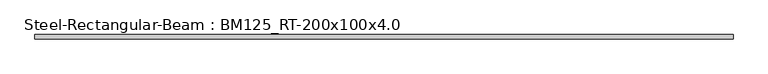
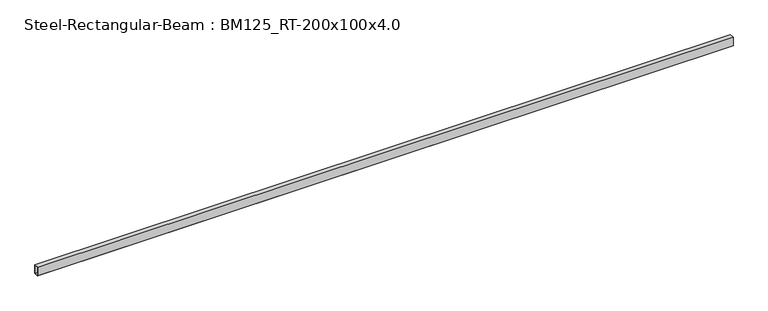
"""IFC4 building model written with IfcOpenShell, lengths in millimetres: beam geometry, Steel-Rectangular-Beam : BM125_RT-200x100x4.0."""

import ifcopenshell
import ifcopenshell.guid

model = None  # the IFC model being written
_history = None  # IfcOwnerHistory: only IFC2X3 demands one
_inside = {}  # id of a spatial element -> (the spatial element, [elements in it])
_under = {}  # id of a project, library or spatial element -> (it, [spatial elements below it])
_declared = {}  # id of a project -> (the project, [libraries it declares])
_typed = {}  # id of a type object -> (the type object, [elements of that type])
_made_of = {}  # id of a material, layer set ... -> (it, [elements and type objects made of it])


def new_model(schema):
    """Start an empty IFC model of exactly this schema.

    Asked for "IFC4X3", IfcOpenShell would pick the latest addendum, in which some entities
    have other attributes; the version numbers below select the first issue.
    IFC2X3 requires an IfcOwnerHistory on every rooted entity: one is made here for all.
    """
    global model, _history
    if schema == "IFC4X3":
        model = ifcopenshell.file(schema_version=(4, 3, 0, 0))
    else:
        model = ifcopenshell.file(schema=schema)
    _inside.clear()
    _under.clear()
    _declared.clear()
    _typed.clear()
    _made_of.clear()
    _history = None
    if model.schema == "IFC2X3":
        org = make("IfcOrganization", Name="unknown")
        user = make(
            "IfcPersonAndOrganization",
            ThePerson=make("IfcPerson", FamilyName="unknown"),
            TheOrganization=org,
        )
        app = make(
            "IfcApplication",
            ApplicationDeveloper=org,
            Version="unknown",
            ApplicationFullName="unknown",
            ApplicationIdentifier="unknown",
        )
        _history = make(
            "IfcOwnerHistory",
            OwningUser=user,
            OwningApplication=app,
            ChangeAction="ADDED",
            CreationDate=0,
        )
    return model


def make(cls, **values):
    """One entity of the class cls with the attributes given. An attribute that is None is left unset."""
    return model.create_entity(
        cls, **{name: value for name, value in values.items() if value is not None}
    )


def rooted(cls, **values):
    """An entity with a GlobalId (a new one), such as an element, a storey or a relation."""
    return make(cls, GlobalId=ifcopenshell.guid.new(), OwnerHistory=_history, **values)


def si_unit(unit_type, name, prefix=None):
    """IfcSIUnit, for example si_unit("LENGTHUNIT", "METRE", prefix="MILLI")."""
    return make("IfcSIUnit", UnitType=unit_type, Prefix=prefix, Name=name)


def assignment(units):
    """IfcUnitAssignment: the units of a project."""
    return None if units is None else make("IfcUnitAssignment", Units=units)


def point(xyz):
    """IfcCartesianPoint."""
    return None if xyz is None else make("IfcCartesianPoint", Coordinates=xyz)


def direction(xyz):
    """IfcDirection."""
    return None if xyz is None else make("IfcDirection", DirectionRatios=xyz)


def frame(location, z_axis=None, x_axis=None):
    """IfcAxis2Placement3D, a coordinate frame: its origin and axes. An axis left out is left unset."""
    return make(
        "IfcAxis2Placement3D",
        Location=point(location),
        Axis=direction(z_axis),
        RefDirection=direction(x_axis),
    )


def origin():
    """The frame at (0, 0, 0) with its axes left unset."""
    return frame((0.0, 0.0, 0.0))


def place(relative_to, where):
    """IfcLocalPlacement: puts the frame where relative to a parent placement (None: the world)."""
    return make(
        "IfcLocalPlacement", PlacementRelTo=relative_to, RelativePlacement=where
    )


def context(
    kind, dimensions, precision=None, world=None, true_north=None, identifier=None
):
    """IfcGeometricRepresentationContext, for example the 3D "Model" context."""
    return make(
        "IfcGeometricRepresentationContext",
        ContextIdentifier=identifier,
        ContextType=kind,
        CoordinateSpaceDimension=dimensions,
        Precision=precision,
        WorldCoordinateSystem=world,
        TrueNorth=true_north,
    )


def project(units=None, contexts=None):
    """IfcProject with its units and contexts."""
    return rooted(
        "IfcProject",
        Name="project",
        RepresentationContexts=contexts,
        UnitsInContext=assignment(units),
    )


def spatial(cls, under=None, at=None, **own):
    """A site, building, storey or space (cls), placed at a placement, below another one or the project."""
    s = rooted(cls, ObjectPlacement=at, **own)
    if under is not None:
        _under.setdefault(under.id(), (under, []))[1].append(s)
    return s


def polyline(points):
    """IfcPolyline through the points."""
    return make("IfcPolyline", Points=[point(p) for p in points])


def outline(outer, holes=None, kind="AREA"):
    """IfcArbitraryClosedProfileDef: a profile drawn as a closed curve; with holes, ...WithVoids."""
    if holes is None:
        return make("IfcArbitraryClosedProfileDef", ProfileType=kind, OuterCurve=outer)
    return make(
        "IfcArbitraryProfileDefWithVoids",
        ProfileType=kind,
        OuterCurve=outer,
        InnerCurves=holes,
    )


def extrude(swept, where, along, depth):
    """IfcExtrudedAreaSolid: the profile swept, set in the frame where, extruded along a direction by depth."""
    return make(
        "IfcExtrudedAreaSolid",
        SweptArea=swept,
        Position=where,
        ExtrudedDirection=direction(along),
        Depth=depth,
    )


def shape(context_of_items, identifier, shape_type, items):
    """IfcShapeRepresentation: the items that make up one representation, for example the "Body"."""
    return make(
        "IfcShapeRepresentation",
        ContextOfItems=context_of_items,
        RepresentationIdentifier=identifier,
        RepresentationType=shape_type,
        Items=items,
    )


def source(mapping_origin, context_of_items, identifier, shape_type, items):
    """IfcRepresentationMap: a shape defined once, which mapped items show again and again."""
    return make(
        "IfcRepresentationMap",
        MappingOrigin=mapping_origin,
        MappedRepresentation=shape(context_of_items, identifier, shape_type, items),
    )


def transform(
    local_origin,
    x_axis=None,
    y_axis=None,
    z_axis=None,
    scale=None,
    scale2=None,
    scale3=None,
    uniform=True,
):
    """IfcCartesianTransformationOperator3D, or its non-uniform kind. x_axis, y_axis, z_axis: its Axis1, 2, 3."""
    if uniform:
        return make(
            "IfcCartesianTransformationOperator3D",
            Axis1=direction(x_axis),
            Axis2=direction(y_axis),
            LocalOrigin=point(local_origin),
            Scale=scale,
            Axis3=direction(z_axis),
        )
    return make(
        "IfcCartesianTransformationOperator3DnonUniform",
        Axis1=direction(x_axis),
        Axis2=direction(y_axis),
        LocalOrigin=point(local_origin),
        Scale=scale,
        Axis3=direction(z_axis),
        Scale2=scale2,
        Scale3=scale3,
    )


def mapped(mapping_source, mapping_target):
    """IfcMappedItem: shows the shape of a source again, moved by a transform."""
    return make(
        "IfcMappedItem", MappingSource=mapping_source, MappingTarget=mapping_target
    )


def made_of(thing, what):
    """Note that an element or type object is made of a material, layer set ...; save() writes the relation."""
    if what is not None:
        _made_of.setdefault(what.id(), (what, []))[1].append(thing)
    return thing


def element(
    cls,
    number,
    at=None,
    inside=None,
    cuts=None,
    type_object=None,
    material=None,
    context=None,
    identifier="Body",
    shape_type=None,
    held_by="IfcProductDefinitionShape",
    body=None,
    shapes=None,
    **own,
):
    """One element of the class cls, such as IfcWall. Its Tag is "e" and its number.

    at: its placement. inside: the storey or other place that contains it. cuts: it is an
    opening in that element (IfcRelVoidsElement). A single representation is given by context,
    identifier, shape_type and body (its items); several are given by shapes. held_by: the class
    of the entity that holds the representations. save() writes the other relations.
    """
    e = rooted(cls, Tag="e%d" % number, ObjectPlacement=at, **own)
    if body is not None:
        shapes = [shape(context, identifier, shape_type, body)]
    if shapes is not None:
        e.Representation = make(held_by, Representations=shapes)
    if inside is not None:
        _inside.setdefault(inside.id(), (inside, []))[1].append(e)
    if cuts is not None:
        rooted(
            "IfcRelVoidsElement", RelatingBuildingElement=cuts, RelatedOpeningElement=e
        )
    if type_object is not None:
        _typed.setdefault(type_object.id(), (type_object, []))[1].append(e)
    return made_of(e, material)


def aggregate(whole, parts):
    """IfcRelAggregates: a whole, such as a stair, and the parts it consists of."""
    return rooted("IfcRelAggregates", RelatingObject=whole, RelatedObjects=parts)


def save(model, path):
    """Write the relations noted so far, then the file.

    IfcRelAggregates (storeys below a building ...), IfcRelContainedInSpatialStructure (elements
    in a storey), IfcRelDefinesByType, IfcRelAssociatesMaterial and IfcRelDeclares: one each for
    every whole, place, type object, material and project.
    """
    for whole, parts in _under.values():
        aggregate(whole, parts)
    for where, things in _inside.values():
        rooted(
            "IfcRelContainedInSpatialStructure",
            RelatedElements=things,
            RelatingStructure=where,
        )
    for kind, things in _typed.values():
        rooted("IfcRelDefinesByType", RelatedObjects=things, RelatingType=kind)
    for what, things in _made_of.values():
        rooted("IfcRelAssociatesMaterial", RelatedObjects=things, RelatingMaterial=what)
    for by, libraries in _declared.values():
        rooted("IfcRelDeclares", RelatingContext=by, RelatedDefinitions=libraries)
    model.write(path)


def steel_rectangular_beam_bm125_rt_200x100x4_0_de2c2afd(model_context):
    return source(origin(), model_context, "Body", "SweptSolid", [
        extrude(outline(polyline([(50.0, 100.0), (50.0, -100.0), (-50.0, -100.0), (-50.0, 100.0), (50.0, 100.0)]), holes=[polyline([(-46.0, -96.0), (46.0, -96.0), (46.0, 96.0), (-46.0, 96.0), (-46.0, -96.0)])]), frame((-7500.0, 0.0, 0.0), z_axis=(1.0, 0.0, 0.0), x_axis=(0.0, 1.0, 0.0)), (0.0, 0.0, 1.0), 15500.0),
        extrude(outline(polyline([(50.0, 100.0), (50.0, -100.0), (-50.0, -100.0), (-50.0, 100.0), (50.0, 100.0)]), holes=[polyline([(-46.0, -96.0), (46.0, -96.0), (46.0, 96.0), (-46.0, 96.0), (-46.0, -96.0)])]), frame((-7500.0, 0.0, 0.0), z_axis=(1.0, 0.0, 0.0), x_axis=(0.0, 1.0, 0.0)), (0.0, 0.0, 1.0), 15500.0),
        extrude(outline(polyline([(50.0, 100.0), (50.0, -100.0), (-50.0, -100.0), (-50.0, 100.0), (50.0, 100.0)]), holes=[polyline([(-46.0, -96.0), (46.0, -96.0), (46.0, 96.0), (-46.0, 96.0), (-46.0, -96.0)])]), frame((-7500.0, 0.0, 0.0), z_axis=(1.0, 0.0, 0.0), x_axis=(0.0, 1.0, 0.0)), (0.0, 0.0, 1.0), 15500.0),
        extrude(outline(polyline([(50.0, 100.0), (50.0, -100.0), (-50.0, -100.0), (-50.0, 100.0), (50.0, 100.0)]), holes=[polyline([(-46.0, -96.0), (46.0, -96.0), (46.0, 96.0), (-46.0, 96.0), (-46.0, -96.0)])]), frame((-7500.0, 0.0, 0.0), z_axis=(1.0, 0.0, 0.0), x_axis=(0.0, 1.0, 0.0)), (0.0, 0.0, 1.0), 15500.0),
    ])


if __name__ == "__main__":
    model = new_model("IFC4")
    model_context = context("Model", 3, world=origin())
    ifc_project = project(units=[si_unit("LENGTHUNIT", "METRE", prefix="MILLI")], contexts=[model_context])
    site = spatial("IfcSite", under=ifc_project)
    building = spatial("IfcBuilding", under=site)
    placement = place(None, origin())
    steel_rectangular_beam_bm125_rt_200x100x4_0_shape = steel_rectangular_beam_bm125_rt_200x100x4_0_de2c2afd(model_context)
    element("IfcBeam", 1, ObjectType="Steel-Rectangular-Beam : BM125_RT-200x100x4.0", at=placement, inside=building, context=model_context, shape_type="MappedRepresentation", body=[
        mapped(steel_rectangular_beam_bm125_rt_200x100x4_0_shape, transform((0.0, 0.0, 0.0), x_axis=(1.0, 0.0, 0.0), y_axis=(0.0, 1.0, 0.0), z_axis=(0.0, 0.0, 1.0))),
    ])
    save(model, "model.ifc")

# Revit data of these elements
# Type "Steel-Rectangular-Beam : BM125_RT-200x100x4.0"
#   t = 4 mm
#   Mass per Unit Length = 18.35 kg/m
#   Surface Area = 0.60 m²/m
#   Sectional Area = 1856.0 cm²
#   Length [instance default] = 3000 mm
#   H = 200 mm
#   B = 100 mm
#   hec_material4 [instance default] = none
#   hec_material3 [instance default] = none
#   hec_material2 [instance default] = none
#   hec_material1 [instance default] = none
#   Structural Material [instance default] = none
# Element 1 (IfcBeam, "Steel-Rectangular-Beam : BM125_RT-200x100x4.0")
#   hec_material2 = S01AA010-00001_Main Steel Structure Fabrication Work_Shelter/Building_Steel Painting/Coating_for Non-Fireproofed Steel Surface, Surface Preparation, Primer, Second & Final Coat
#   hec_material1 = S03AA007-00001_Main Steel Structure Erection Work_Girth & Purlin
#   Structural Material = S01AA007-00001_Main Steel Structure Fabrication Work_Shelter/Building_Girth & Purlin
#   Materials on its faces: "S01AA010-00001_Main Steel Structure Fabrication Work_Shelter/Building_Steel Painting/Coating_for Non-Fireproofed Steel Surface, Surface Preparation, Primer, Second & Final Coat"
# Materials
#   "S01AA010-00001_Main Steel Structure Fabrication Work_Shelter/Building_Steel Painting/Coating_for Non-Fireproofed Steel Surface, Surface Preparation, Primer, Second & Final Coat": class "Metal", colour RGB 120 120 120, transparency 0, Description = "Paint finished steel", W00) Work Master Code = "S01AA010-00001", W01) Work Master_Lv1 = "Main Steel Structure Fabrication Work", W02) Work Master_Lv2 = "Shelter/Building", W03) Work Master_Spec.1 = "Steel Painting/Coating", W04) Work Master_Spec.2 = "for Non-Fireproofed Steel Surface, Surface Preparation, Primer, Second & Final Coat", Cost = 0
#   "S03AA007-00001_Main Steel Structure Erection Work_Girth & Purlin": class "Metal", colour RGB 120 120 120, transparency 0, Comments = "(30KG/M>Weight)", Description = "Structural steel 50ksi", W00) Work Master Code = "S03AA007-00001", W01) Work Master_Lv1 = "Main Steel Structure Erection Work", W02) Work Master_Lv2 = "Shelter/Building", W03) Work Master_Spec.1 = "Girth & Purlin", Cost = 0
#   "S01AA007-00001_Main Steel Structure Fabrication Work_Shelter/Building_Girth & Purlin": class "Metal", colour RGB 120 120 120, transparency 0, Comments = "(30KG/M>Weight)", Description = "Structural steel 50ksi", W00) Work Master Code = "S01AA007-00001", W01) Work Master_Lv1 = "Main Steel Structure Fabrication Work", W02) Work Master_Lv2 = "Shelter/Building", W03) Work Master_Spec.1 = "Girth & Purlin", Cost = 0
